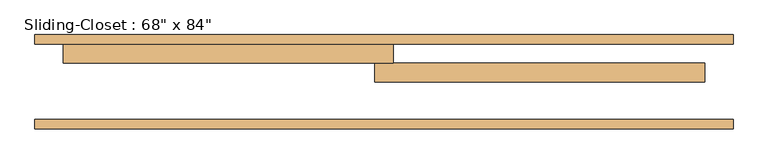
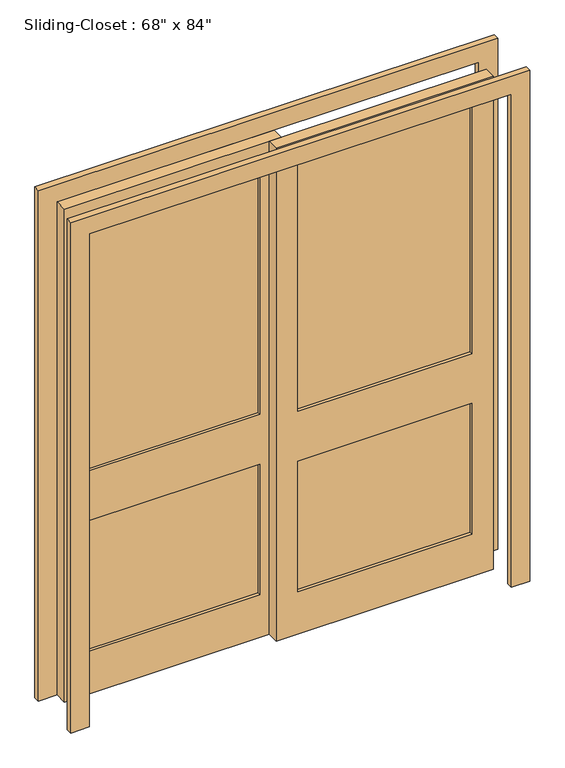
"""IFC4 building model written with IfcOpenShell, lengths in millimetres: door geometry."""

from ifc_helpers import new_model, si_unit, frame, origin, place, context, project, spatial, polyline, outline, extrude, source, transform, mapped, element, save


def door_2f313a91(model_context):
    return source(origin(), model_context, "Body", "SweptSolid", [
        extrude(outline(polyline([(-63.5, 190.5), (-774.7, 190.5), (-774.7, 215.9), (-63.5, 215.9), (-63.5, 190.5)])), frame((0.0, 0.0, 965.2), z_axis=(0.0, 0.0, 1.0), x_axis=(1.0, 0.0, 0.0)), (0.0, 0.0, 1.0), 1079.5),
        extrude(outline(polyline([(-63.5, 190.5), (-774.7, 190.5), (-774.7, 215.9), (-63.5, 215.9), (-63.5, 190.5)])), frame((0.0, 0.0, 184.15), z_axis=(0.0, 0.0, 1.0), x_axis=(1.0, 0.0, 0.0)), (0.0, 0.0, 1.0), 565.15),
        extrude(outline(polyline([(63.5, 165.1), (774.7, 165.1), (774.7, 139.7), (63.5, 139.7), (63.5, 165.1)])), frame((0.0, 0.0, 965.2), z_axis=(0.0, 0.0, 1.0), x_axis=(1.0, 0.0, 0.0)), (0.0, 0.0, 1.0), 1079.5),
        extrude(outline(polyline([(63.5, 165.1), (774.7, 165.1), (774.7, 139.7), (63.5, 139.7), (63.5, 165.1)])), frame((0.0, 0.0, 184.15), z_axis=(0.0, 0.0, 1.0), x_axis=(1.0, 0.0, 0.0)), (0.0, 0.0, 1.0), 565.15),
        extrude(outline(polyline([(2133.6, 25.4), (2133.6, -863.6), (0.0, -863.6), (0.0, 25.4), (2133.6, 25.4)]), holes=[polyline([(184.15, -774.7), (749.3, -774.7), (749.3, -63.5), (184.15, -63.5), (184.15, -774.7)]), polyline([(965.2, -774.7), (2044.7, -774.7), (2044.7, -63.5), (965.2, -63.5), (965.2, -774.7)])]), frame((0.0, 177.8, 0.0), z_axis=(0.0, 1.0, 0.0), x_axis=(0.0, 0.0, 1.0)), (0.0, 0.0, 1.0), 50.8),
        extrude(outline(polyline([(0.0, -939.8), (0.0, -863.6), (2133.6, -863.6), (2133.6, 863.6), (0.0, 863.6), (0.0, 939.8), (2209.8, 939.8), (2209.8, -939.8), (0.0, -939.8)])), frame((0.0, 0.0, 0.0), z_axis=(0.0, 1.0, 0.0), x_axis=(0.0, 0.0, 1.0)), (0.0, 0.0, 1.0), 25.4),
        extrude(outline(polyline([(0.0, 939.8), (2209.8, 939.8), (2209.8, -939.8), (0.0, -939.8), (0.0, -863.6), (2133.6, -863.6), (2133.6, 863.6), (0.0, 863.6), (0.0, 939.8)])), frame((0.0, 228.6, 0.0), z_axis=(0.0, 1.0, 0.0), x_axis=(0.0, 0.0, 1.0)), (0.0, 0.0, 1.0), 25.4),
        extrude(outline(polyline([(2133.6, -25.4), (0.0, -25.4), (0.0, 863.6), (2133.6, 863.6), (2133.6, -25.4)]), holes=[polyline([(965.2, 774.7), (965.2, 63.5), (2044.7, 63.5), (2044.7, 774.7), (965.2, 774.7)]), polyline([(184.15, 774.7), (184.15, 63.5), (749.3, 63.5), (749.3, 774.7), (184.15, 774.7)])]), frame((0.0, 127.0, 0.0), z_axis=(0.0, 1.0, 0.0), x_axis=(0.0, 0.0, 1.0)), (0.0, 0.0, 1.0), 50.8),
    ])


if __name__ == "__main__":
    model = new_model("IFC4")
    model_context = context("Model", 3, world=origin())
    ifc_project = project(units=[si_unit("LENGTHUNIT", "METRE", prefix="MILLI")], contexts=[model_context])
    site = spatial("IfcSite", under=ifc_project)
    building = spatial("IfcBuilding", under=site)
    placement = place(None, origin())
    door_shape = door_2f313a91(model_context)
    element("IfcDoor", 1, ObjectType="Sliding-Closet : 68\" x 84\"", at=placement, inside=building, context=model_context, shape_type="MappedRepresentation", body=[
        mapped(door_shape, transform((0.0, 0.0, 0.0), x_axis=(1.0, 0.0, 0.0), y_axis=(0.0, 1.0, 0.0), z_axis=(0.0, 0.0, 1.0))),
    ])
    save(model, "model.ifc")

# Revit data of these elements
# Type "Sliding-Closet : 68\" x 84\""
#   Type Mark = "50"
#   Assembly Code = "C1020"
#   Thickness = 0' - 2"
#   Height = 7' - 0"
#   Trim Projection Ext = 0' - 1"
#   Trim Projection Int = 0' - 1"
#   Trim Width = 0' - 3"
#   Width = 5' - 8"
#   Define Thermal Properties by = 0
#   Function = 0
#   Door Material = Door - Panel
#   Frame Material = Door - Frame
#   Wall Closure = (empty or 0)
# Element 1 (IfcDoor, "Sliding-Closet : 68\" x 84\"")
#   Materials on its faces: "Door - Panel", "Door - Frame"
# Materials
#   "Door - Panel": class "Wood", colour RGB 227 170 128, transparency 0, Cost = 0
#   "Door - Frame": class "Miscellaneous", colour RGB 153 76 43, transparency 0, Cost = 0
